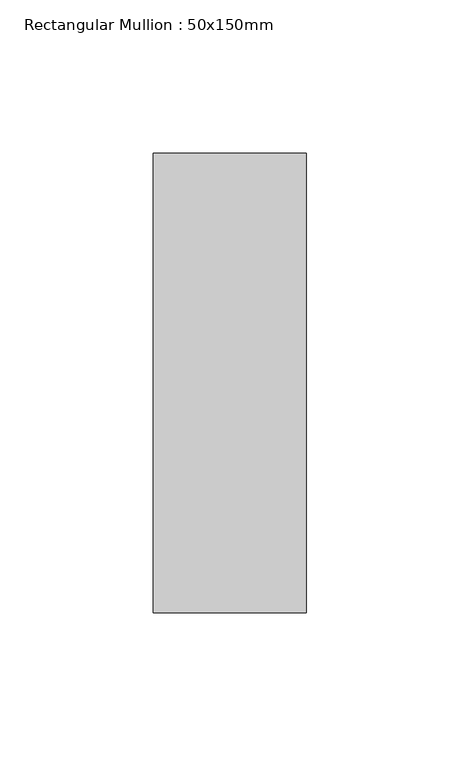
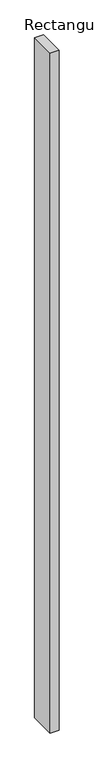
"""IFC4 building model written with IfcOpenShell, lengths in millimetres: member geometry, Rectangular Mullion : 50x150mm."""

from ifc_helpers import new_model, si_unit, frame, origin, place, context, project, spatial, polyline, outline, extrude, source, transform, mapped, element, save


def rectangular_mullion_50x150mm_0357f134(model_context):
    return source(origin(), model_context, "Body", "SweptSolid", [
        extrude(outline(polyline([(0.0, 75.0), (0.0, -75.0), (-50.0, -75.0), (-50.0, 75.0), (0.0, 75.0)])), frame((0.0, 0.0, -4000.0), z_axis=(0.0, 0.0, 1.0), x_axis=(1.0, 0.0, 0.0)), (0.0, 0.0, 1.0), 4000.0),
    ])


if __name__ == "__main__":
    model = new_model("IFC4")
    model_context = context("Model", 3, world=origin())
    ifc_project = project(units=[si_unit("LENGTHUNIT", "METRE", prefix="MILLI")], contexts=[model_context])
    site = spatial("IfcSite", under=ifc_project)
    building = spatial("IfcBuilding", under=site)
    placement = place(None, origin())
    rectangular_mullion_50x150mm_shape = rectangular_mullion_50x150mm_0357f134(model_context)
    element("IfcMember", 1, ObjectType="Rectangular Mullion : 50x150mm", at=placement, inside=building, context=model_context, shape_type="MappedRepresentation", body=[
        mapped(rectangular_mullion_50x150mm_shape, transform((0.0, 0.0, 0.0), x_axis=(1.0, 0.0, 0.0), y_axis=(0.0, 1.0, 0.0), z_axis=(0.0, 0.0, 1.0))),
    ])
    save(model, "model.ifc")

# Revit data of these elements
# Project information
#   Project Issue Date = "Issue Date"
#   Project Status = "Project Status"
#   Client Name = "Owner"
#   Project Address = "Enter address here"
#   Project Name = "Project Name"
#   Project Number = "Project Number"
# Type "Rectangular Mullion : 50x150mm"
#   Keynote = "H11"
#   built-in parameter 1007304 = 0.492126 (stored number, unit not read)
#   built-in parameter 1007301 = 0.082021 (stored number, unit not read)
#   built-in parameter 1007300 = 0.082021 (stored number, unit not read)
# Element 1 (IfcMember, "Rectangular Mullion : 50x150mm")
#   Materials on its faces: "Aluminium"
# Materials
#   "Aluminium": class "Metal", colour RGB 247 247 247, transparency 0, Description = "Aluminium 6061", Cost = 0
